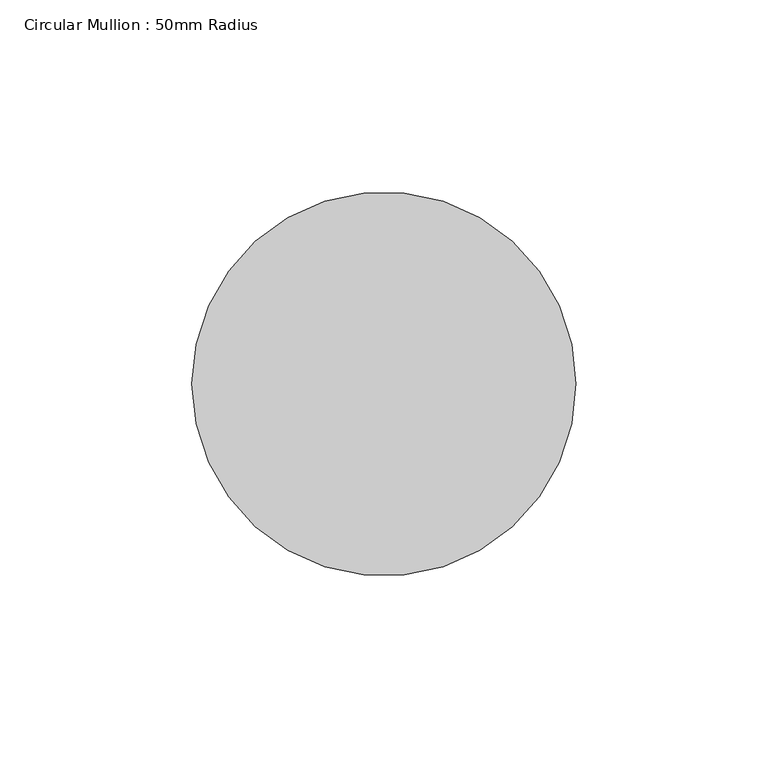
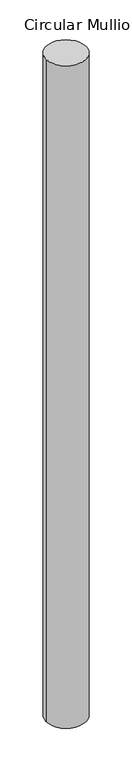
"""IFC4 building model written with IfcOpenShell, lengths in millimetres: member geometry, Circular Mullion : 50mm Radius."""

from ifc_helpers import new_model, si_unit, point, frame, frame_2d, origin, place, context, project, spatial, circle_curve, trimmed, segment, composite_curve, outline, extrude, source, transform, mapped, element, save


def circular_mullion_50mm_radius_63d095c5(model_context):
    return source(origin(), model_context, "Body", "SweptSolid", [
        extrude(outline(composite_curve([segment(trimmed(circle_curve(frame_2d((-50.0, 0.0)), 50.0), [point((0.0, 0.0))], [point((-100.0, 0.0))], False, "CARTESIAN"), True, "CONTINUOUS"), segment(trimmed(circle_curve(frame_2d((-50.0, 0.0)), 50.0), [point((-100.0, 0.0))], [point((0.0, 0.0))], False, "CARTESIAN"), True, "CONTINUOUS")], self_intersect=False)), frame((0.0, 0.0, -1764.2243777), z_axis=(0.0, 0.0, 1.0), x_axis=(1.0, 0.0, 0.0)), (0.0, 0.0, 1.0), 1764.2243777),
    ])


if __name__ == "__main__":
    model = new_model("IFC4")
    model_context = context("Model", 3, world=origin())
    ifc_project = project(units=[si_unit("LENGTHUNIT", "METRE", prefix="MILLI")], contexts=[model_context])
    site = spatial("IfcSite", under=ifc_project)
    building = spatial("IfcBuilding", under=site)
    placement = place(None, origin())
    circular_mullion_50mm_radius_shape = circular_mullion_50mm_radius_63d095c5(model_context)
    element("IfcMember", 1, ObjectType="Circular Mullion : 50mm Radius", at=placement, inside=building, context=model_context, shape_type="MappedRepresentation", body=[
        mapped(circular_mullion_50mm_radius_shape, transform((0.0, 0.0, 0.0), x_axis=(1.0, 0.0, 0.0), y_axis=(0.0, 1.0, 0.0), z_axis=(0.0, 0.0, 1.0))),
    ])
    save(model, "model.ifc")

# Revit data of these elements
# Type "Circular Mullion : 50mm Radius"
#   built-in parameter 1007350 = 0.164042 (stored number, unit not read)
# Element 1 (IfcMember, "Circular Mullion : 50mm Radius")
#   Materials on its faces: "Aluminium"
# Materials
#   "Aluminium": class "Metal", colour RGB 247 247 247, transparency 0, Description = "Aluminium 6061", Cost = 0
